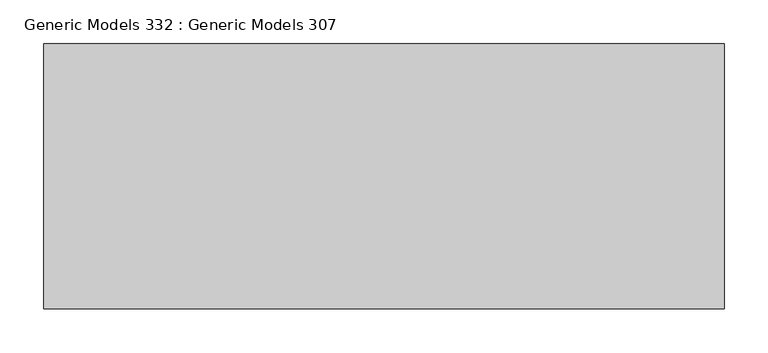
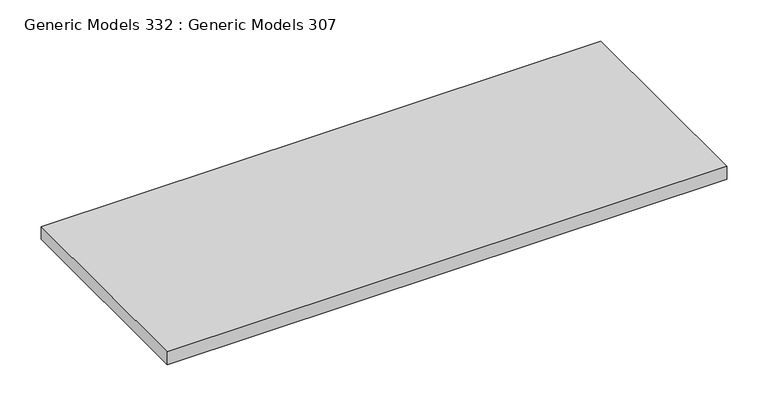
"""IFC4 building model written with IfcOpenShell, lengths in millimetres: proxy geometry, Generic Models 332 : Generic Models 307."""

from ifc_helpers import new_model, si_unit, frame, origin, place, context, project, spatial, polyline, outline, extrude, source, transform, mapped, element, save


def generic_models_332_generic_models_307_19b28fce(model_context):
    return source(origin(), model_context, "Body", "SweptSolid", [
        extrude(outline(polyline([(4057.4763704, 704.5309662), (4839.3786898, 704.5309662), (4839.3786898, 399.7309662), (4057.4763704, 399.7309662), (4057.4763704, 704.5309662)])), frame((0.0, 0.0, 129209.546), z_axis=(0.0, 0.0, 1.0), x_axis=(1.0, 0.0, 0.0)), (0.0, 0.0, 1.0), 19.05),
    ])


if __name__ == "__main__":
    model = new_model("IFC4")
    model_context = context("Model", 3, world=origin())
    ifc_project = project(units=[si_unit("LENGTHUNIT", "METRE", prefix="MILLI")], contexts=[model_context])
    site = spatial("IfcSite", under=ifc_project)
    building = spatial("IfcBuilding", under=site)
    placement = place(None, origin())
    generic_models_332_generic_models_307_shape = generic_models_332_generic_models_307_19b28fce(model_context)
    element("IfcBuildingElementProxy", 1, Name="Generic Models 332 : Generic Models 307", ObjectType="Generic Models 332 : Generic Models 307", at=placement, inside=building, context=model_context, shape_type="MappedRepresentation", body=[
        mapped(generic_models_332_generic_models_307_shape, transform((0.0, 0.0, 0.0), x_axis=(1.0, 0.0, 0.0), y_axis=(0.0, 1.0, 0.0), z_axis=(0.0, 0.0, 1.0))),
    ])
    save(model, "model.ifc")

# Revit data of these elements
# Element 1 (IfcBuildingElementProxy, "Generic Models 332 : Generic Models 307")
#   Materials on its faces: "_WOOD CEILING (SPEC T.B.D.)"
# Materials
#   "_WOOD CEILING (SPEC T.B.D.)": class "Generic", colour RGB 177 130 114, transparency 0, Cost = 0
